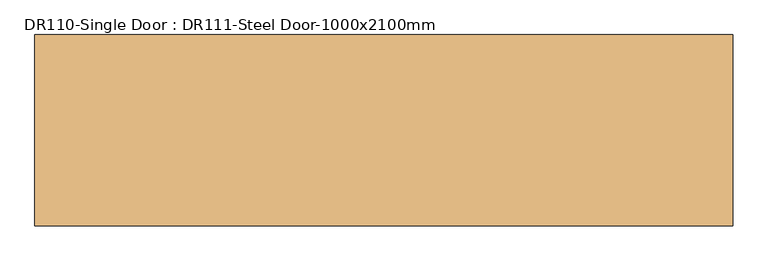
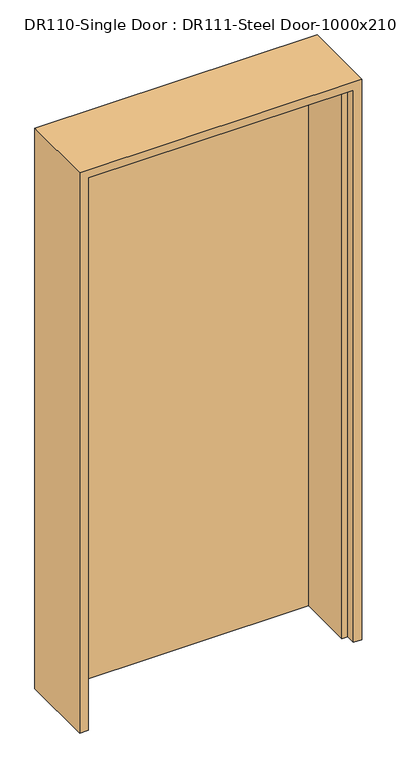
"""IFC4 building model written with IfcOpenShell, lengths in millimetres: door geometry, DR110-Single Door : DR111-Steel Door-1000x2100mm."""

from ifc_helpers import new_model, si_unit, origin, origin_with_axes, place, context, project, spatial, polyline, outline, extrude, faceted_brep, source, transform, mapped, element, save


def dr110_single_door_dr111_steel_door_1000x2100mm_d0b51d4b(model_context):
    return source(origin(), model_context, "Body", "SolidModel", [
        extrude(outline(polyline([(470.0, 137.0), (470.0, 102.0), (-470.0, 102.0), (-470.0, 137.0), (470.0, 137.0)])), origin_with_axes(), (0.0, 0.0, 1.0), 2070.0),
        faceted_brep([(470.0, 137.0, 0.0), (500.0, 137.0, 0.0), (500.0, -137.0, 0.0), (470.0, -137.0, 0.0), (470.0, -102.0, 0.0), (450.0, -102.0, 0.0), (450.0, 102.0, 0.0), (470.0, 102.0, 0.0), (470.0, 137.0, 2070.0), (-470.0, 137.0, 2070.0), (-470.0, 137.0, 0.0), (-500.0, 137.0, 0.0), (-500.0, 137.0, 2100.0), (500.0, 137.0, 2100.0), (500.0, -137.0, 2100.0), (-500.0, -137.0, 2100.0), (-500.0, -137.0, 0.0), (-470.0, -137.0, 0.0), (-470.0, -137.0, 2070.0), (470.0, -137.0, 2070.0), (470.0, -102.0, 2070.0), (-470.0, -102.0, 2070.0), (-470.0, -102.0, 0.0), (-450.0, -102.0, 0.0), (-450.0, -102.0, 2050.0), (450.0, -102.0, 2050.0), (450.0, 102.0, 2050.0), (-450.0, 102.0, 2050.0), (-450.0, 102.0, 0.0), (-470.0, 102.0, 0.0), (-470.0, 102.0, 2070.0), (470.0, 102.0, 2070.0)], [[[0, 1, 2, 3, 4, 5, 6, 7]], [[1, 0, 8, 9, 10, 11, 12, 13]], [[2, 1, 13, 14]], [[3, 2, 14, 15, 16, 17, 18, 19]], [[4, 3, 19, 20]], [[5, 4, 20, 21, 22, 23, 24, 25]], [[6, 5, 25, 26]], [[7, 6, 26, 27, 28, 29, 30, 31]], [[0, 7, 31, 8]], [[9, 30, 29, 10]], [[10, 29, 28, 23, 22, 17, 16, 11]], [[15, 12, 11, 16]], [[21, 18, 17, 22]], [[27, 24, 23, 28]], [[14, 13, 12, 15]], [[20, 19, 18, 21]], [[26, 25, 24, 27]], [[8, 31, 30, 9]]]),
    ])


if __name__ == "__main__":
    model = new_model("IFC4")
    model_context = context("Model", 3, world=origin())
    ifc_project = project(units=[si_unit("LENGTHUNIT", "METRE", prefix="MILLI")], contexts=[model_context])
    site = spatial("IfcSite", under=ifc_project)
    building = spatial("IfcBuilding", under=site)
    placement = place(None, origin())
    dr110_single_door_dr111_steel_door_1000x2100mm_shape = dr110_single_door_dr111_steel_door_1000x2100mm_d0b51d4b(model_context)
    element("IfcDoor", 1, ObjectType="DR110-Single Door : DR111-Steel Door-1000x2100mm", at=placement, inside=building, context=model_context, shape_type="MappedRepresentation", body=[
        mapped(dr110_single_door_dr111_steel_door_1000x2100mm_shape, transform((0.0, 0.0, 0.0), x_axis=(1.0, 0.0, 0.0), y_axis=(0.0, 1.0, 0.0), z_axis=(0.0, 0.0, 1.0))),
    ])
    save(model, "model.ifc")

# Revit data of these elements
# Type "DR110-Single Door : DR111-Steel Door-1000x2100mm"
#   Type Mark = "SD"
#   Analytic Construction = "<None>"
#   프레임 투영 외부. = 25 mm
#   프레임 투영 내부. = 25 mm
#   프레임 폭 = 75 mm
#   Height = 2100 mm
#   Width = 1000 mm
#   Define Thermal Properties by = 1
#   문 패널 = SD1 문 패널
#   문 프레임 = A04AQ098-00002_Steel Door_non FP_single
#   Function = (empty or 0)
#   Wall Closure = (empty or 0)
# Element 1 (IfcDoor, "DR110-Single Door : DR111-Steel Door-1000x2100mm")
#   Materials on its faces: "A04AQ098-00002_Steel Door_non FP_single", "SD1 문 패널"
# Materials
#   "SD1 문 패널": class "금속", colour RGB 247 247 247, transparency 0, Description = "STEEL DOOR (1000Wx2100H)"
#   "A04AQ098-00002_Steel Door_non FP_single": class "금속", colour RGB 247 247 247, transparency 0, Description = "Steel Door", W00) Work Master Code = "A04AQ098-00002", W01) Work Master_Lv1 = "Finishing Work", W02) Work Master_Lv2 = "Door & Window Work", W03) Work Master_Spec.1 = "Steel Door w/ Steel Frame", W04) Work Master_Spec.2 = "Fire Protective Rating: N/A, Single Door", W05) Work Master_Spec.3 = "w/ Hardware & Accessories", Cost = 0
